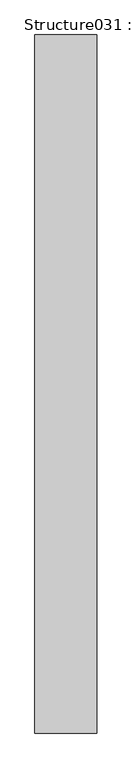
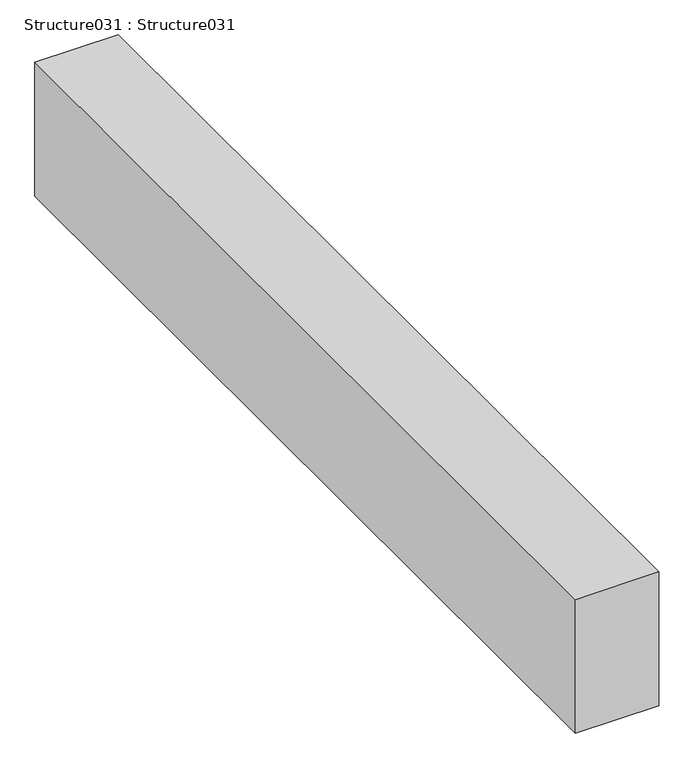
"""IFC4 building model written with IfcOpenShell, lengths in millimetres: proxy geometry, Structure031 : Structure031."""

import ifcopenshell
import ifcopenshell.guid

model = None  # the IFC model being written
_history = None  # IfcOwnerHistory: only IFC2X3 demands one
_inside = {}  # id of a spatial element -> (the spatial element, [elements in it])
_under = {}  # id of a project, library or spatial element -> (it, [spatial elements below it])
_declared = {}  # id of a project -> (the project, [libraries it declares])
_typed = {}  # id of a type object -> (the type object, [elements of that type])
_made_of = {}  # id of a material, layer set ... -> (it, [elements and type objects made of it])


def new_model(schema):
    """Start an empty IFC model of exactly this schema.

    Asked for "IFC4X3", IfcOpenShell would pick the latest addendum, in which some entities
    have other attributes; the version numbers below select the first issue.
    IFC2X3 requires an IfcOwnerHistory on every rooted entity: one is made here for all.
    """
    global model, _history
    if schema == "IFC4X3":
        model = ifcopenshell.file(schema_version=(4, 3, 0, 0))
    else:
        model = ifcopenshell.file(schema=schema)
    _inside.clear()
    _under.clear()
    _declared.clear()
    _typed.clear()
    _made_of.clear()
    _history = None
    if model.schema == "IFC2X3":
        org = make("IfcOrganization", Name="unknown")
        user = make(
            "IfcPersonAndOrganization",
            ThePerson=make("IfcPerson", FamilyName="unknown"),
            TheOrganization=org,
        )
        app = make(
            "IfcApplication",
            ApplicationDeveloper=org,
            Version="unknown",
            ApplicationFullName="unknown",
            ApplicationIdentifier="unknown",
        )
        _history = make(
            "IfcOwnerHistory",
            OwningUser=user,
            OwningApplication=app,
            ChangeAction="ADDED",
            CreationDate=0,
        )
    return model


def make(cls, **values):
    """One entity of the class cls with the attributes given. An attribute that is None is left unset."""
    return model.create_entity(
        cls, **{name: value for name, value in values.items() if value is not None}
    )


def rooted(cls, **values):
    """An entity with a GlobalId (a new one), such as an element, a storey or a relation."""
    return make(cls, GlobalId=ifcopenshell.guid.new(), OwnerHistory=_history, **values)


def si_unit(unit_type, name, prefix=None):
    """IfcSIUnit, for example si_unit("LENGTHUNIT", "METRE", prefix="MILLI")."""
    return make("IfcSIUnit", UnitType=unit_type, Prefix=prefix, Name=name)


def assignment(units):
    """IfcUnitAssignment: the units of a project."""
    return None if units is None else make("IfcUnitAssignment", Units=units)


def point(xyz):
    """IfcCartesianPoint."""
    return None if xyz is None else make("IfcCartesianPoint", Coordinates=xyz)


def direction(xyz):
    """IfcDirection."""
    return None if xyz is None else make("IfcDirection", DirectionRatios=xyz)


def frame(location, z_axis=None, x_axis=None):
    """IfcAxis2Placement3D, a coordinate frame: its origin and axes. An axis left out is left unset."""
    return make(
        "IfcAxis2Placement3D",
        Location=point(location),
        Axis=direction(z_axis),
        RefDirection=direction(x_axis),
    )


def origin():
    """The frame at (0, 0, 0) with its axes left unset."""
    return frame((0.0, 0.0, 0.0))


def place(relative_to, where):
    """IfcLocalPlacement: puts the frame where relative to a parent placement (None: the world)."""
    return make(
        "IfcLocalPlacement", PlacementRelTo=relative_to, RelativePlacement=where
    )


def context(
    kind, dimensions, precision=None, world=None, true_north=None, identifier=None
):
    """IfcGeometricRepresentationContext, for example the 3D "Model" context."""
    return make(
        "IfcGeometricRepresentationContext",
        ContextIdentifier=identifier,
        ContextType=kind,
        CoordinateSpaceDimension=dimensions,
        Precision=precision,
        WorldCoordinateSystem=world,
        TrueNorth=true_north,
    )


def project(units=None, contexts=None):
    """IfcProject with its units and contexts."""
    return rooted(
        "IfcProject",
        Name="project",
        RepresentationContexts=contexts,
        UnitsInContext=assignment(units),
    )


def spatial(cls, under=None, at=None, **own):
    """A site, building, storey or space (cls), placed at a placement, below another one or the project."""
    s = rooted(cls, ObjectPlacement=at, **own)
    if under is not None:
        _under.setdefault(under.id(), (under, []))[1].append(s)
    return s


def polyline(points):
    """IfcPolyline through the points."""
    return make("IfcPolyline", Points=[point(p) for p in points])


def outline(outer, holes=None, kind="AREA"):
    """IfcArbitraryClosedProfileDef: a profile drawn as a closed curve; with holes, ...WithVoids."""
    if holes is None:
        return make("IfcArbitraryClosedProfileDef", ProfileType=kind, OuterCurve=outer)
    return make(
        "IfcArbitraryProfileDefWithVoids",
        ProfileType=kind,
        OuterCurve=outer,
        InnerCurves=holes,
    )


def extrude(swept, where, along, depth):
    """IfcExtrudedAreaSolid: the profile swept, set in the frame where, extruded along a direction by depth."""
    return make(
        "IfcExtrudedAreaSolid",
        SweptArea=swept,
        Position=where,
        ExtrudedDirection=direction(along),
        Depth=depth,
    )


def shape(context_of_items, identifier, shape_type, items):
    """IfcShapeRepresentation: the items that make up one representation, for example the "Body"."""
    return make(
        "IfcShapeRepresentation",
        ContextOfItems=context_of_items,
        RepresentationIdentifier=identifier,
        RepresentationType=shape_type,
        Items=items,
    )


def source(mapping_origin, context_of_items, identifier, shape_type, items):
    """IfcRepresentationMap: a shape defined once, which mapped items show again and again."""
    return make(
        "IfcRepresentationMap",
        MappingOrigin=mapping_origin,
        MappedRepresentation=shape(context_of_items, identifier, shape_type, items),
    )


def transform(
    local_origin,
    x_axis=None,
    y_axis=None,
    z_axis=None,
    scale=None,
    scale2=None,
    scale3=None,
    uniform=True,
):
    """IfcCartesianTransformationOperator3D, or its non-uniform kind. x_axis, y_axis, z_axis: its Axis1, 2, 3."""
    if uniform:
        return make(
            "IfcCartesianTransformationOperator3D",
            Axis1=direction(x_axis),
            Axis2=direction(y_axis),
            LocalOrigin=point(local_origin),
            Scale=scale,
            Axis3=direction(z_axis),
        )
    return make(
        "IfcCartesianTransformationOperator3DnonUniform",
        Axis1=direction(x_axis),
        Axis2=direction(y_axis),
        LocalOrigin=point(local_origin),
        Scale=scale,
        Axis3=direction(z_axis),
        Scale2=scale2,
        Scale3=scale3,
    )


def mapped(mapping_source, mapping_target):
    """IfcMappedItem: shows the shape of a source again, moved by a transform."""
    return make(
        "IfcMappedItem", MappingSource=mapping_source, MappingTarget=mapping_target
    )


def made_of(thing, what):
    """Note that an element or type object is made of a material, layer set ...; save() writes the relation."""
    if what is not None:
        _made_of.setdefault(what.id(), (what, []))[1].append(thing)
    return thing


def element(
    cls,
    number,
    at=None,
    inside=None,
    cuts=None,
    type_object=None,
    material=None,
    context=None,
    identifier="Body",
    shape_type=None,
    held_by="IfcProductDefinitionShape",
    body=None,
    shapes=None,
    **own,
):
    """One element of the class cls, such as IfcWall. Its Tag is "e" and its number.

    at: its placement. inside: the storey or other place that contains it. cuts: it is an
    opening in that element (IfcRelVoidsElement). A single representation is given by context,
    identifier, shape_type and body (its items); several are given by shapes. held_by: the class
    of the entity that holds the representations. save() writes the other relations.
    """
    e = rooted(cls, Tag="e%d" % number, ObjectPlacement=at, **own)
    if body is not None:
        shapes = [shape(context, identifier, shape_type, body)]
    if shapes is not None:
        e.Representation = make(held_by, Representations=shapes)
    if inside is not None:
        _inside.setdefault(inside.id(), (inside, []))[1].append(e)
    if cuts is not None:
        rooted(
            "IfcRelVoidsElement", RelatingBuildingElement=cuts, RelatedOpeningElement=e
        )
    if type_object is not None:
        _typed.setdefault(type_object.id(), (type_object, []))[1].append(e)
    return made_of(e, material)


def aggregate(whole, parts):
    """IfcRelAggregates: a whole, such as a stair, and the parts it consists of."""
    return rooted("IfcRelAggregates", RelatingObject=whole, RelatedObjects=parts)


def save(model, path):
    """Write the relations noted so far, then the file.

    IfcRelAggregates (storeys below a building ...), IfcRelContainedInSpatialStructure (elements
    in a storey), IfcRelDefinesByType, IfcRelAssociatesMaterial and IfcRelDeclares: one each for
    every whole, place, type object, material and project.
    """
    for whole, parts in _under.values():
        aggregate(whole, parts)
    for where, things in _inside.values():
        rooted(
            "IfcRelContainedInSpatialStructure",
            RelatedElements=things,
            RelatingStructure=where,
        )
    for kind, things in _typed.values():
        rooted("IfcRelDefinesByType", RelatedObjects=things, RelatingType=kind)
    for what, things in _made_of.values():
        rooted("IfcRelAssociatesMaterial", RelatedObjects=things, RelatingMaterial=what)
    for by, libraries in _declared.values():
        rooted("IfcRelDeclares", RelatingContext=by, RelatedDefinitions=libraries)
    model.write(path)


def structure031_structure031_ec718016(model_context):
    return source(origin(), model_context, "Body", "SweptSolid", [
        extrude(outline(polyline([(-6778.6276325, 7982.1531721), (-6956.4276325, 7982.1531721), (-6956.4276325, 9982.1531721), (-6778.6276325, 9982.1531721), (-6778.6276325, 7982.1531721)])), frame((0.0, 0.0, 39579.2960083), z_axis=(0.0, 0.0, 1.0), x_axis=(1.0, 0.0, 0.0)), (0.0, 0.0, 1.0), 301.625),
    ])


if __name__ == "__main__":
    model = new_model("IFC4")
    model_context = context("Model", 3, world=origin())
    ifc_project = project(units=[si_unit("LENGTHUNIT", "METRE", prefix="MILLI")], contexts=[model_context])
    site = spatial("IfcSite", under=ifc_project)
    building = spatial("IfcBuilding", under=site)
    placement = place(None, origin())
    structure031_structure031_shape = structure031_structure031_ec718016(model_context)
    element("IfcBuildingElementProxy", 1, Name="Structure031 : Structure031", ObjectType="Structure031 : Structure031", at=placement, inside=building, context=model_context, shape_type="MappedRepresentation", body=[
        mapped(structure031_structure031_shape, transform((0.0, 0.0, 0.0), x_axis=(1.0, 0.0, 0.0), y_axis=(0.0, 1.0, 0.0), z_axis=(0.0, 0.0, 1.0))),
    ])
    save(model, "model.ifc")

# Revit data of these elements
# Type "Structure031 : Structure031"
#   NameOverride = "Structure031"
# Element 1 (IfcBuildingElementProxy, "Structure031 : Structure031")
#   Materials on its faces: "STRUCTURAL MEMBER (SEE STRUCTURAL DWGS)"
# Materials
#   "STRUCTURAL MEMBER (SEE STRUCTURAL DWGS)": class "Unassigned", colour RGB 176 134 95, transparency 0, Cost = 0
